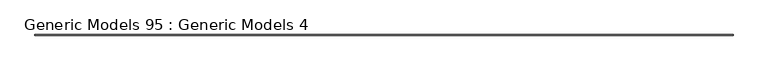
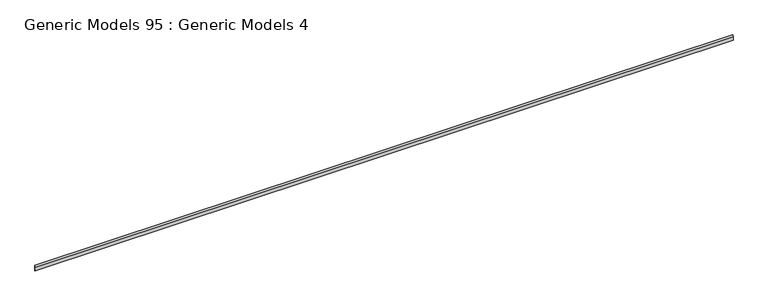
"""IFC4 building model written with IfcOpenShell, lengths in millimetres: proxy geometry, Generic Models 95 : Generic Models 4."""

from ifc_helpers import new_model, si_unit, frame, origin, place, context, project, spatial, polyline, outline, extrude, source, transform, mapped, element, save


def generic_models_95_generic_models_4_0415544c(model_context):
    return source(origin(), model_context, "Body", "SweptSolid", [
        extrude(outline(polyline([(51457.9426718, 127006.935011), (51457.9426718, 127109.3314334), (51475.7226718, 127143.9556439), (51475.7226718, 127001.220011), (51457.9426718, 127006.935011)])), frame((-20795.7733045, 0.0, 0.0), z_axis=(1.0, 0.0, 0.0), x_axis=(0.0, 1.0, 0.0)), (0.0, 0.0, 1.0), 18643.6),
    ])


if __name__ == "__main__":
    model = new_model("IFC4")
    model_context = context("Model", 3, world=origin())
    ifc_project = project(units=[si_unit("LENGTHUNIT", "METRE", prefix="MILLI")], contexts=[model_context])
    site = spatial("IfcSite", under=ifc_project)
    building = spatial("IfcBuilding", under=site)
    placement = place(None, origin())
    generic_models_95_generic_models_4_shape = generic_models_95_generic_models_4_0415544c(model_context)
    element("IfcBuildingElementProxy", 1, Name="Generic Models 95 : Generic Models 4", ObjectType="Generic Models 95 : Generic Models 4", at=placement, inside=building, context=model_context, shape_type="MappedRepresentation", body=[
        mapped(generic_models_95_generic_models_4_shape, transform((0.0, 0.0, 0.0), x_axis=(1.0, 0.0, 0.0), y_axis=(0.0, 1.0, 0.0), z_axis=(0.0, 0.0, 1.0))),
    ])
    save(model, "model.ifc")

# Revit data of these elements
# Element 1 (IfcBuildingElementProxy, "Generic Models 95 : Generic Models 4")
#   Materials on its faces: "_7/8\" SMOOTH TROWEL EXTERIOR STUCCO (COLOR PER OWNER)"
# Materials
#   "_7/8\" SMOOTH TROWEL EXTERIOR STUCCO (COLOR PER OWNER)": class "Generic", colour RGB 233 233 233, transparency 0, Cost = 0
